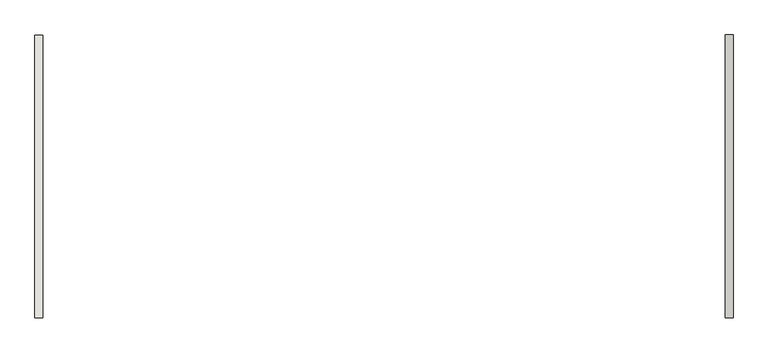
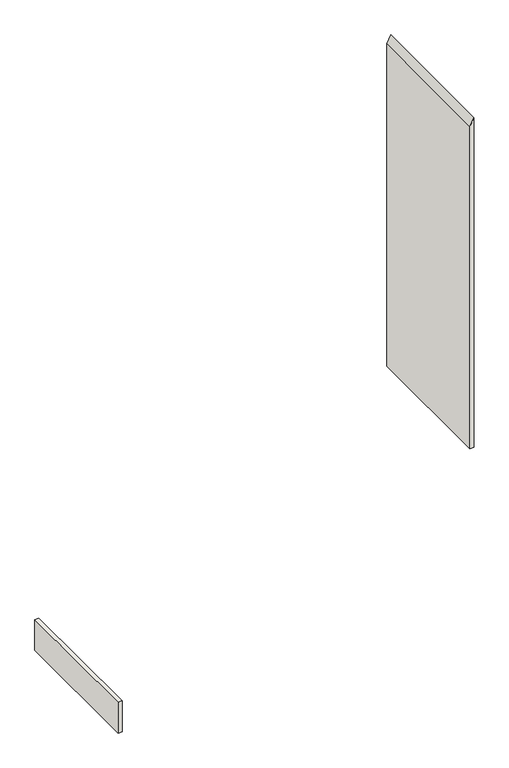
"""IFC4 building model written with IfcOpenShell, lengths in millimetres: wall geometry, WOOD SIDING - T.B.D. : WOOD SIDING - T.B.D.."""

import ifcopenshell
import ifcopenshell.guid

model = None  # the IFC model being written
_history = None  # IfcOwnerHistory: only IFC2X3 demands one
_inside = {}  # id of a spatial element -> (the spatial element, [elements in it])
_under = {}  # id of a project, library or spatial element -> (it, [spatial elements below it])
_declared = {}  # id of a project -> (the project, [libraries it declares])
_typed = {}  # id of a type object -> (the type object, [elements of that type])
_made_of = {}  # id of a material, layer set ... -> (it, [elements and type objects made of it])


def new_model(schema):
    """Start an empty IFC model of exactly this schema.

    Asked for "IFC4X3", IfcOpenShell would pick the latest addendum, in which some entities
    have other attributes; the version numbers below select the first issue.
    IFC2X3 requires an IfcOwnerHistory on every rooted entity: one is made here for all.
    """
    global model, _history
    if schema == "IFC4X3":
        model = ifcopenshell.file(schema_version=(4, 3, 0, 0))
    else:
        model = ifcopenshell.file(schema=schema)
    _inside.clear()
    _under.clear()
    _declared.clear()
    _typed.clear()
    _made_of.clear()
    _history = None
    if model.schema == "IFC2X3":
        org = make("IfcOrganization", Name="unknown")
        user = make(
            "IfcPersonAndOrganization",
            ThePerson=make("IfcPerson", FamilyName="unknown"),
            TheOrganization=org,
        )
        app = make(
            "IfcApplication",
            ApplicationDeveloper=org,
            Version="unknown",
            ApplicationFullName="unknown",
            ApplicationIdentifier="unknown",
        )
        _history = make(
            "IfcOwnerHistory",
            OwningUser=user,
            OwningApplication=app,
            ChangeAction="ADDED",
            CreationDate=0,
        )
    return model


def make(cls, **values):
    """One entity of the class cls with the attributes given. An attribute that is None is left unset."""
    return model.create_entity(
        cls, **{name: value for name, value in values.items() if value is not None}
    )


def rooted(cls, **values):
    """An entity with a GlobalId (a new one), such as an element, a storey or a relation."""
    return make(cls, GlobalId=ifcopenshell.guid.new(), OwnerHistory=_history, **values)


def si_unit(unit_type, name, prefix=None):
    """IfcSIUnit, for example si_unit("LENGTHUNIT", "METRE", prefix="MILLI")."""
    return make("IfcSIUnit", UnitType=unit_type, Prefix=prefix, Name=name)


def assignment(units):
    """IfcUnitAssignment: the units of a project."""
    return None if units is None else make("IfcUnitAssignment", Units=units)


def point(xyz):
    """IfcCartesianPoint."""
    return None if xyz is None else make("IfcCartesianPoint", Coordinates=xyz)


def direction(xyz):
    """IfcDirection."""
    return None if xyz is None else make("IfcDirection", DirectionRatios=xyz)


def frame(location, z_axis=None, x_axis=None):
    """IfcAxis2Placement3D, a coordinate frame: its origin and axes. An axis left out is left unset."""
    return make(
        "IfcAxis2Placement3D",
        Location=point(location),
        Axis=direction(z_axis),
        RefDirection=direction(x_axis),
    )


def origin():
    """The frame at (0, 0, 0) with its axes left unset."""
    return frame((0.0, 0.0, 0.0))


def place(relative_to, where):
    """IfcLocalPlacement: puts the frame where relative to a parent placement (None: the world)."""
    return make(
        "IfcLocalPlacement", PlacementRelTo=relative_to, RelativePlacement=where
    )


def context(
    kind, dimensions, precision=None, world=None, true_north=None, identifier=None
):
    """IfcGeometricRepresentationContext, for example the 3D "Model" context."""
    return make(
        "IfcGeometricRepresentationContext",
        ContextIdentifier=identifier,
        ContextType=kind,
        CoordinateSpaceDimension=dimensions,
        Precision=precision,
        WorldCoordinateSystem=world,
        TrueNorth=true_north,
    )


def project(units=None, contexts=None):
    """IfcProject with its units and contexts."""
    return rooted(
        "IfcProject",
        Name="project",
        RepresentationContexts=contexts,
        UnitsInContext=assignment(units),
    )


def spatial(cls, under=None, at=None, **own):
    """A site, building, storey or space (cls), placed at a placement, below another one or the project."""
    s = rooted(cls, ObjectPlacement=at, **own)
    if under is not None:
        _under.setdefault(under.id(), (under, []))[1].append(s)
    return s


def polyline(points):
    """IfcPolyline through the points."""
    return make("IfcPolyline", Points=[point(p) for p in points])


def outline(outer, holes=None, kind="AREA"):
    """IfcArbitraryClosedProfileDef: a profile drawn as a closed curve; with holes, ...WithVoids."""
    if holes is None:
        return make("IfcArbitraryClosedProfileDef", ProfileType=kind, OuterCurve=outer)
    return make(
        "IfcArbitraryProfileDefWithVoids",
        ProfileType=kind,
        OuterCurve=outer,
        InnerCurves=holes,
    )


def extrude(swept, where, along, depth):
    """IfcExtrudedAreaSolid: the profile swept, set in the frame where, extruded along a direction by depth."""
    return make(
        "IfcExtrudedAreaSolid",
        SweptArea=swept,
        Position=where,
        ExtrudedDirection=direction(along),
        Depth=depth,
    )


def shape(context_of_items, identifier, shape_type, items):
    """IfcShapeRepresentation: the items that make up one representation, for example the "Body"."""
    return make(
        "IfcShapeRepresentation",
        ContextOfItems=context_of_items,
        RepresentationIdentifier=identifier,
        RepresentationType=shape_type,
        Items=items,
    )


def source(mapping_origin, context_of_items, identifier, shape_type, items):
    """IfcRepresentationMap: a shape defined once, which mapped items show again and again."""
    return make(
        "IfcRepresentationMap",
        MappingOrigin=mapping_origin,
        MappedRepresentation=shape(context_of_items, identifier, shape_type, items),
    )


def transform(
    local_origin,
    x_axis=None,
    y_axis=None,
    z_axis=None,
    scale=None,
    scale2=None,
    scale3=None,
    uniform=True,
):
    """IfcCartesianTransformationOperator3D, or its non-uniform kind. x_axis, y_axis, z_axis: its Axis1, 2, 3."""
    if uniform:
        return make(
            "IfcCartesianTransformationOperator3D",
            Axis1=direction(x_axis),
            Axis2=direction(y_axis),
            LocalOrigin=point(local_origin),
            Scale=scale,
            Axis3=direction(z_axis),
        )
    return make(
        "IfcCartesianTransformationOperator3DnonUniform",
        Axis1=direction(x_axis),
        Axis2=direction(y_axis),
        LocalOrigin=point(local_origin),
        Scale=scale,
        Axis3=direction(z_axis),
        Scale2=scale2,
        Scale3=scale3,
    )


def mapped(mapping_source, mapping_target):
    """IfcMappedItem: shows the shape of a source again, moved by a transform."""
    return make(
        "IfcMappedItem", MappingSource=mapping_source, MappingTarget=mapping_target
    )


def made_of(thing, what):
    """Note that an element or type object is made of a material, layer set ...; save() writes the relation."""
    if what is not None:
        _made_of.setdefault(what.id(), (what, []))[1].append(thing)
    return thing


def element(
    cls,
    number,
    at=None,
    inside=None,
    cuts=None,
    type_object=None,
    material=None,
    context=None,
    identifier="Body",
    shape_type=None,
    held_by="IfcProductDefinitionShape",
    body=None,
    shapes=None,
    **own,
):
    """One element of the class cls, such as IfcWall. Its Tag is "e" and its number.

    at: its placement. inside: the storey or other place that contains it. cuts: it is an
    opening in that element (IfcRelVoidsElement). A single representation is given by context,
    identifier, shape_type and body (its items); several are given by shapes. held_by: the class
    of the entity that holds the representations. save() writes the other relations.
    """
    e = rooted(cls, Tag="e%d" % number, ObjectPlacement=at, **own)
    if body is not None:
        shapes = [shape(context, identifier, shape_type, body)]
    if shapes is not None:
        e.Representation = make(held_by, Representations=shapes)
    if inside is not None:
        _inside.setdefault(inside.id(), (inside, []))[1].append(e)
    if cuts is not None:
        rooted(
            "IfcRelVoidsElement", RelatingBuildingElement=cuts, RelatedOpeningElement=e
        )
    if type_object is not None:
        _typed.setdefault(type_object.id(), (type_object, []))[1].append(e)
    return made_of(e, material)


def aggregate(whole, parts):
    """IfcRelAggregates: a whole, such as a stair, and the parts it consists of."""
    return rooted("IfcRelAggregates", RelatingObject=whole, RelatedObjects=parts)


def save(model, path):
    """Write the relations noted so far, then the file.

    IfcRelAggregates (storeys below a building ...), IfcRelContainedInSpatialStructure (elements
    in a storey), IfcRelDefinesByType, IfcRelAssociatesMaterial and IfcRelDeclares: one each for
    every whole, place, type object, material and project.
    """
    for whole, parts in _under.values():
        aggregate(whole, parts)
    for where, things in _inside.values():
        rooted(
            "IfcRelContainedInSpatialStructure",
            RelatedElements=things,
            RelatingStructure=where,
        )
    for kind, things in _typed.values():
        rooted("IfcRelDefinesByType", RelatedObjects=things, RelatingType=kind)
    for what, things in _made_of.values():
        rooted("IfcRelAssociatesMaterial", RelatedObjects=things, RelatingMaterial=what)
    for by, libraries in _declared.values():
        rooted("IfcRelDeclares", RelatingContext=by, RelatedDefinitions=libraries)
    model.write(path)


def wall_0c4a4a7f(model_context):
    return source(origin(), model_context, "Body", "SweptSolid", [
        extrude(outline(polyline([(17895.2878203, -2319.6634634), (17876.2378203, -2319.6634634), (17876.2378203, -1633.8634634), (17895.2878203, -1633.8634634), (17895.2878203, -2319.6634634)])), frame((0.0, 0.0, 2198.6875), z_axis=(0.0, 0.0, 1.0), x_axis=(1.0, 0.0, 0.0)), (0.0, 0.0, 1.0), 154.9707982),
        extrude(outline(polyline([(4661.2557155, 19550.4587335), (3041.7352617, 19550.4587335), (3041.7352617, 19569.5087335), (4699.3557155, 19569.5087335), (4661.2557155, 19550.4587335)])), frame((0.0, -2319.6634634, 0.0), z_axis=(0.0, 1.0, 0.0), x_axis=(0.0, 0.0, 1.0)), (0.0, 0.0, 1.0), 685.8),
    ])


if __name__ == "__main__":
    model = new_model("IFC4")
    model_context = context("Model", 3, world=origin())
    ifc_project = project(units=[si_unit("LENGTHUNIT", "METRE", prefix="MILLI")], contexts=[model_context])
    site = spatial("IfcSite", under=ifc_project)
    building = spatial("IfcBuilding", under=site)
    placement = place(None, origin())
    wall_shape = wall_0c4a4a7f(model_context)
    element("IfcWall", 1, ObjectType="WOOD SIDING - T.B.D. : WOOD SIDING - T.B.D.", at=placement, inside=building, context=model_context, shape_type="MappedRepresentation", body=[
        mapped(wall_shape, transform((0.0, 0.0, 0.0), x_axis=(1.0, 0.0, 0.0), y_axis=(0.0, 1.0, 0.0), z_axis=(0.0, 0.0, 1.0))),
    ])
    save(model, "model.ifc")

# Revit data of these elements
# Element 1 (IfcWall, "WOOD SIDING - T.B.D. : WOOD SIDING - T.B.D.")
#   Materials on its faces: "WOOD SIDING - T.B.D."
# Materials
#   "WOOD SIDING - T.B.D.": class "Generic", colour RGB 234 234 234, transparency 0, Cost = 0
